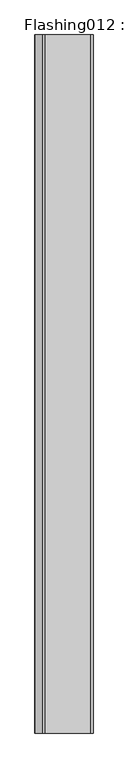
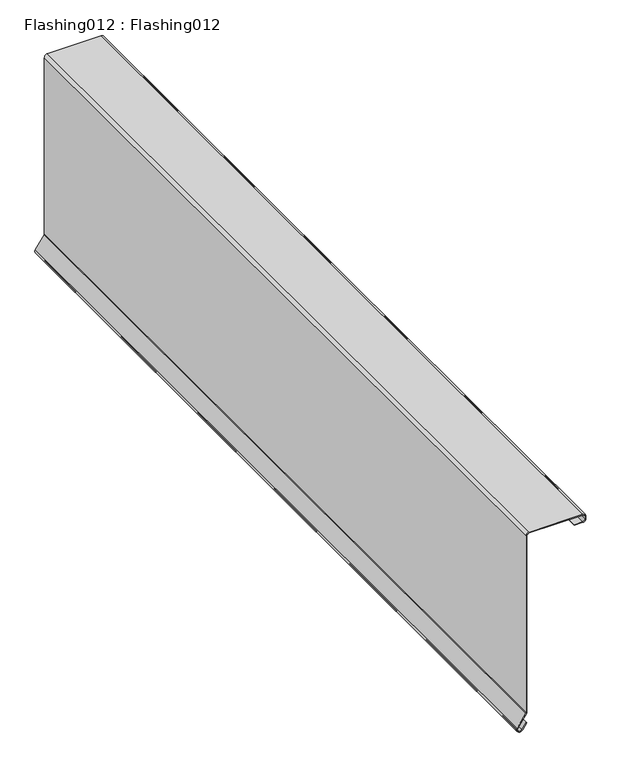
"""IFC4 building model written with IfcOpenShell, lengths in millimetres: proxy geometry, Flashing012 : Flashing012."""

from ifc_helpers import new_model, si_unit, point, frame, frame_2d, origin, place, context, project, spatial, polyline, circle_curve, trimmed, segment, composite_curve, outline, extrude, source, transform, mapped, element, save


def flashing012_flashing012_affd795f(model_context):
    return source(origin(), model_context, "Body", "SweptSolid", [
        extrude(outline(composite_curve([segment(trimmed(circle_curve(frame_2d((42111.5532705, -2482.9530802)), 5.08), [point((42108.6312101, -2478.7976063))], [point((42107.4417652, -2485.9366895))], True, "CARTESIAN"), True, "CONTINUOUS"), segment(polyline([(42107.4417652, -2485.9366895), (42108.7344443, -2487.718041)]), True, "CONTINUOUS"), segment(trimmed(circle_curve(frame_2d((42112.8459496, -2484.7344317)), 5.08), [point((42108.7344443, -2487.718041))], [point((42115.753039, -2488.9003927))], True, "CARTESIAN"), True, "CONTINUOUS"), segment(polyline([(42115.753039, -2488.9003927), (42146.0058896, -2467.7893589)]), True, "CONTINUOUS"), segment(trimmed(circle_curve(frame_2d((42148.9129791, -2471.9553199)), 5.08), [point((42146.0058896, -2467.7893589))], [point((42148.9129791, -2466.8753199))], False, "CARTESIAN"), True, "CONTINUOUS"), segment(polyline([(42148.9129791, -2466.8753199), (42596.1419896, -2466.8753199)]), True, "CONTINUOUS"), segment(trimmed(circle_curve(frame_2d((42596.1419896, -2461.7953199)), 5.08), [point((42596.1419896, -2466.8753199))], [point((42601.2219896, -2461.7953199))], True, "CARTESIAN"), True, "CONTINUOUS"), segment(polyline([(42601.2219896, -2461.7953199), (42601.2219896, -2332.4553199)]), True, "CONTINUOUS"), segment(trimmed(circle_curve(frame_2d((42596.1419896, -2332.4553199)), 5.08), [point((42601.2219896, -2332.4553199))], [point((42596.1419896, -2327.3753199))], True, "CARTESIAN"), True, "CONTINUOUS"), segment(polyline([(42596.1419896, -2327.3753199), (42589.7355833, -2327.3753199)]), True, "CONTINUOUS"), segment(trimmed(circle_curve(frame_2d((42589.7355833, -2332.4553199)), 5.08), [point((42589.7355833, -2327.3753199))], [point((42584.6555833, -2332.4553199))], True, "CARTESIAN"), True, "CONTINUOUS"), segment(polyline([(42584.6555833, -2332.4553199), (42584.6555833, -2353.7517847), (42582.6555833, -2353.7517847), (42582.6555833, -2332.4553199)]), True, "CONTINUOUS"), segment(trimmed(circle_curve(frame_2d((42589.7355833, -2332.4553199)), 7.08), [point((42582.6555833, -2332.4553199))], [point((42589.7355833, -2325.3753199))], False, "CARTESIAN"), True, "CONTINUOUS"), segment(polyline([(42589.7355833, -2325.3753199), (42596.1419896, -2325.3753199)]), True, "CONTINUOUS"), segment(trimmed(circle_curve(frame_2d((42596.1419896, -2332.4553199)), 7.08), [point((42596.1419896, -2325.3753199))], [point((42603.2219896, -2332.4553199))], False, "CARTESIAN"), True, "CONTINUOUS"), segment(polyline([(42603.2219896, -2332.4553199), (42603.2219896, -2461.7953199)]), True, "CONTINUOUS"), segment(trimmed(circle_curve(frame_2d((42596.1419896, -2461.7953199)), 7.08), [point((42603.2219896, -2461.7953199))], [point((42596.1419896, -2468.8753199))], False, "CARTESIAN"), True, "CONTINUOUS"), segment(polyline([(42596.1419896, -2468.8753199), (42148.9129791, -2468.8753199)]), True, "CONTINUOUS"), segment(trimmed(circle_curve(frame_2d((42148.9129791, -2471.9553199)), 3.08), [point((42148.9129791, -2468.8753199))], [point((42147.150413, -2469.429501))], True, "CARTESIAN"), True, "CONTINUOUS"), segment(polyline([(42147.150413, -2469.429501), (42116.8975624, -2490.5405348)]), True, "CONTINUOUS"), segment(trimmed(circle_curve(frame_2d((42112.8459496, -2484.7344317)), 7.08), [point((42116.8975624, -2490.5405348))], [point((42107.1157415, -2488.8926904))], False, "CARTESIAN"), True, "CONTINUOUS"), segment(polyline([(42107.1157415, -2488.8926904), (42105.8230624, -2487.1113389)]), True, "CONTINUOUS"), segment(trimmed(circle_curve(frame_2d((42111.5532705, -2482.9530802)), 7.08), [point((42105.8230624, -2487.1113389))], [point((42107.4807927, -2477.161593))], False, "CARTESIAN"), True, "CONTINUOUS"), segment(polyline([(42107.4807927, -2477.161593), (42122.0676658, -2466.9043456), (42123.2180833, -2468.5403589), (42108.6312101, -2478.7976063)]), True, "CONTINUOUS")], self_intersect=False)), frame((0.0, -1052.8906574, 0.0), z_axis=(0.0, 1.0, 0.0), x_axis=(0.0, 0.0, 1.0)), (0.0, 0.0, 1.0), 2000.0),
    ])


if __name__ == "__main__":
    model = new_model("IFC4")
    model_context = context("Model", 3, world=origin())
    ifc_project = project(units=[si_unit("LENGTHUNIT", "METRE", prefix="MILLI")], contexts=[model_context])
    site = spatial("IfcSite", under=ifc_project)
    building = spatial("IfcBuilding", under=site)
    placement = place(None, origin())
    flashing012_flashing012_shape = flashing012_flashing012_affd795f(model_context)
    element("IfcBuildingElementProxy", 1, Name="Flashing012 : Flashing012", ObjectType="Flashing012 : Flashing012", at=placement, inside=building, context=model_context, shape_type="MappedRepresentation", body=[
        mapped(flashing012_flashing012_shape, transform((0.0, 0.0, 0.0), x_axis=(1.0, 0.0, 0.0), y_axis=(0.0, 1.0, 0.0), z_axis=(0.0, 0.0, 1.0))),
    ])
    save(model, "model.ifc")

# Revit data of these elements
# Type "Flashing012 : Flashing012"
#   NameOverride = "Flashing012"
# Element 1 (IfcBuildingElementProxy, "Flashing012 : Flashing012")
#   Materials on its faces: "HIGH EAVE FLASHING"
# Materials
#   "HIGH EAVE FLASHING": class "Unassigned", colour RGB 128 128 128, transparency 0
